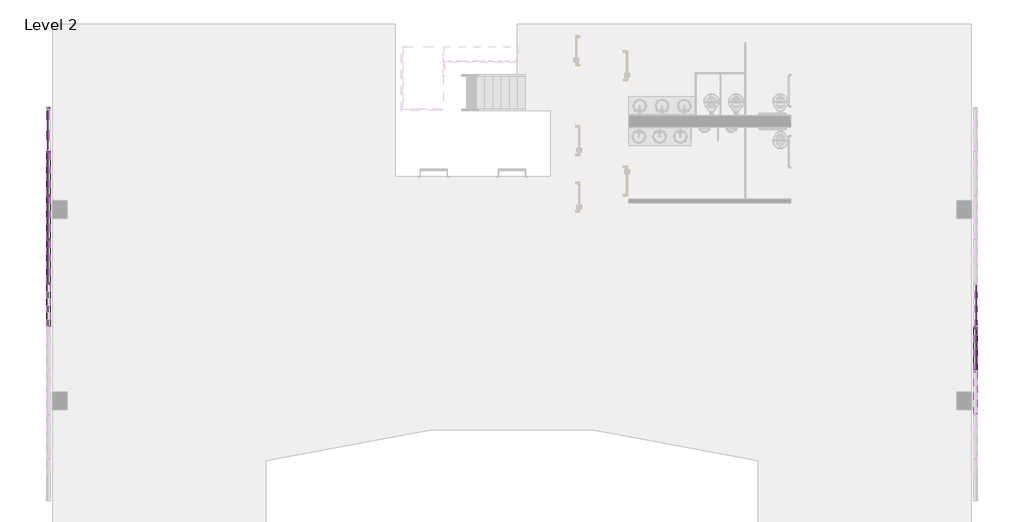
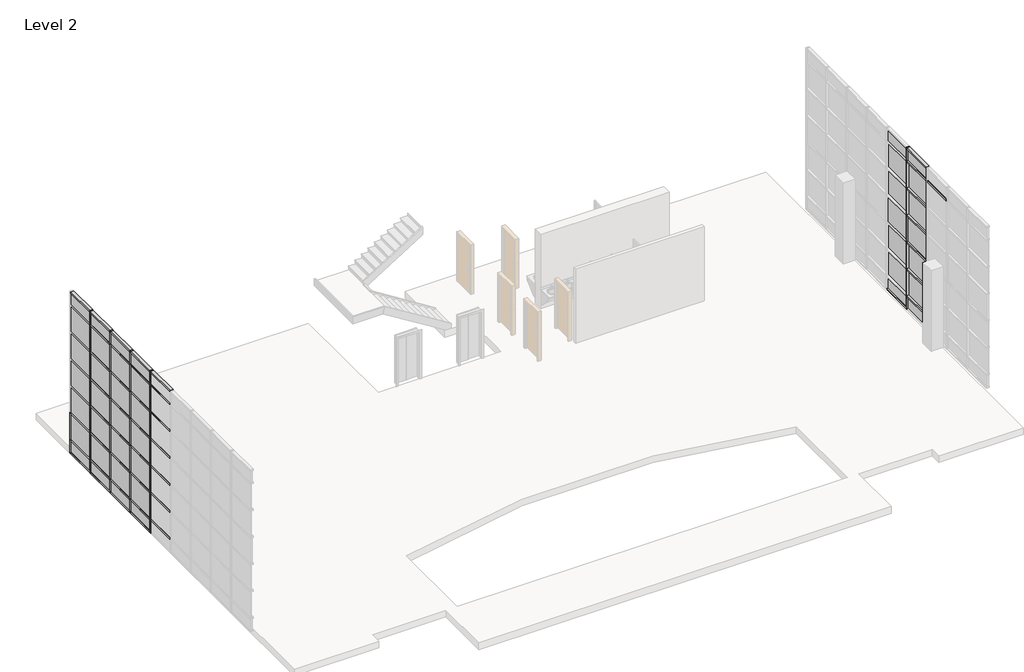
# One storey, part 4 of 6: 79 members, 42 plates.
"""IFC4 building model written with IfcOpenShell, lengths in millimetres."""

import ifcopenshell
import ifcopenshell.guid

model = None  # the IFC model being written
_history = None  # IfcOwnerHistory: only IFC2X3 demands one
_inside = {}  # id of a spatial element -> (the spatial element, [elements in it])
_under = {}  # id of a project, library or spatial element -> (it, [spatial elements below it])
_declared = {}  # id of a project -> (the project, [libraries it declares])
_typed = {}  # id of a type object -> (the type object, [elements of that type])
_made_of = {}  # id of a material, layer set ... -> (it, [elements and type objects made of it])


def new_model(schema):
    """Start an empty IFC model of exactly this schema.

    Asked for "IFC4X3", IfcOpenShell would pick the latest addendum, in which some entities
    have other attributes; the version numbers below select the first issue.
    IFC2X3 requires an IfcOwnerHistory on every rooted entity: one is made here for all.
    """
    global model, _history
    if schema == "IFC4X3":
        model = ifcopenshell.file(schema_version=(4, 3, 0, 0))
    else:
        model = ifcopenshell.file(schema=schema)
    _inside.clear()
    _under.clear()
    _declared.clear()
    _typed.clear()
    _made_of.clear()
    _history = None
    if model.schema == "IFC2X3":
        org = make("IfcOrganization", Name="unknown")
        user = make(
            "IfcPersonAndOrganization",
            ThePerson=make("IfcPerson", FamilyName="unknown"),
            TheOrganization=org,
        )
        app = make(
            "IfcApplication",
            ApplicationDeveloper=org,
            Version="unknown",
            ApplicationFullName="unknown",
            ApplicationIdentifier="unknown",
        )
        _history = make(
            "IfcOwnerHistory",
            OwningUser=user,
            OwningApplication=app,
            ChangeAction="ADDED",
            CreationDate=0,
        )
    return model


def make(cls, **values):
    """One entity of the class cls with the attributes given. An attribute that is None is left unset."""
    return model.create_entity(
        cls, **{name: value for name, value in values.items() if value is not None}
    )


def rooted(cls, **values):
    """An entity with a GlobalId (a new one), such as an element, a storey or a relation."""
    return make(cls, GlobalId=ifcopenshell.guid.new(), OwnerHistory=_history, **values)


def si_unit(unit_type, name, prefix=None):
    """IfcSIUnit, for example si_unit("LENGTHUNIT", "METRE", prefix="MILLI")."""
    return make("IfcSIUnit", UnitType=unit_type, Prefix=prefix, Name=name)


def assignment(units):
    """IfcUnitAssignment: the units of a project."""
    return None if units is None else make("IfcUnitAssignment", Units=units)


def point(xyz):
    """IfcCartesianPoint."""
    return None if xyz is None else make("IfcCartesianPoint", Coordinates=xyz)


def direction(xyz):
    """IfcDirection."""
    return None if xyz is None else make("IfcDirection", DirectionRatios=xyz)


def frame(location, z_axis=None, x_axis=None):
    """IfcAxis2Placement3D, a coordinate frame: its origin and axes. An axis left out is left unset."""
    return make(
        "IfcAxis2Placement3D",
        Location=point(location),
        Axis=direction(z_axis),
        RefDirection=direction(x_axis),
    )


def origin():
    """The frame at (0, 0, 0) with its axes left unset."""
    return frame((0.0, 0.0, 0.0))


def origin_with_axes():
    """The frame at (0, 0, 0) with the z axis (0, 0, 1) and the x axis (1, 0, 0) written out."""
    return frame((0.0, 0.0, 0.0), z_axis=(0.0, 0.0, 1.0), x_axis=(1.0, 0.0, 0.0))


def place(relative_to, where):
    """IfcLocalPlacement: puts the frame where relative to a parent placement (None: the world)."""
    return make(
        "IfcLocalPlacement", PlacementRelTo=relative_to, RelativePlacement=where
    )


def context(
    kind, dimensions, precision=None, world=None, true_north=None, identifier=None
):
    """IfcGeometricRepresentationContext, for example the 3D "Model" context."""
    return make(
        "IfcGeometricRepresentationContext",
        ContextIdentifier=identifier,
        ContextType=kind,
        CoordinateSpaceDimension=dimensions,
        Precision=precision,
        WorldCoordinateSystem=world,
        TrueNorth=true_north,
    )


def project(units=None, contexts=None):
    """IfcProject with its units and contexts."""
    return rooted(
        "IfcProject",
        Name="project",
        RepresentationContexts=contexts,
        UnitsInContext=assignment(units),
    )


def spatial(cls, under=None, at=None, **own):
    """A site, building, storey or space (cls), placed at a placement, below another one or the project."""
    s = rooted(cls, ObjectPlacement=at, **own)
    if under is not None:
        _under.setdefault(under.id(), (under, []))[1].append(s)
    return s


def polyline(points):
    """IfcPolyline through the points."""
    return make("IfcPolyline", Points=[point(p) for p in points])


def outline(outer, holes=None, kind="AREA"):
    """IfcArbitraryClosedProfileDef: a profile drawn as a closed curve; with holes, ...WithVoids."""
    if holes is None:
        return make("IfcArbitraryClosedProfileDef", ProfileType=kind, OuterCurve=outer)
    return make(
        "IfcArbitraryProfileDefWithVoids",
        ProfileType=kind,
        OuterCurve=outer,
        InnerCurves=holes,
    )


def extrude(swept, where, along, depth):
    """IfcExtrudedAreaSolid: the profile swept, set in the frame where, extruded along a direction by depth."""
    return make(
        "IfcExtrudedAreaSolid",
        SweptArea=swept,
        Position=where,
        ExtrudedDirection=direction(along),
        Depth=depth,
    )


def shape(context_of_items, identifier, shape_type, items):
    """IfcShapeRepresentation: the items that make up one representation, for example the "Body"."""
    return make(
        "IfcShapeRepresentation",
        ContextOfItems=context_of_items,
        RepresentationIdentifier=identifier,
        RepresentationType=shape_type,
        Items=items,
    )


def source(mapping_origin, context_of_items, identifier, shape_type, items):
    """IfcRepresentationMap: a shape defined once, which mapped items show again and again."""
    return make(
        "IfcRepresentationMap",
        MappingOrigin=mapping_origin,
        MappedRepresentation=shape(context_of_items, identifier, shape_type, items),
    )


def transform(
    local_origin,
    x_axis=None,
    y_axis=None,
    z_axis=None,
    scale=None,
    scale2=None,
    scale3=None,
    uniform=True,
):
    """IfcCartesianTransformationOperator3D, or its non-uniform kind. x_axis, y_axis, z_axis: its Axis1, 2, 3."""
    if uniform:
        return make(
            "IfcCartesianTransformationOperator3D",
            Axis1=direction(x_axis),
            Axis2=direction(y_axis),
            LocalOrigin=point(local_origin),
            Scale=scale,
            Axis3=direction(z_axis),
        )
    return make(
        "IfcCartesianTransformationOperator3DnonUniform",
        Axis1=direction(x_axis),
        Axis2=direction(y_axis),
        LocalOrigin=point(local_origin),
        Scale=scale,
        Axis3=direction(z_axis),
        Scale2=scale2,
        Scale3=scale3,
    )


def mapped(mapping_source, mapping_target):
    """IfcMappedItem: shows the shape of a source again, moved by a transform."""
    return make(
        "IfcMappedItem", MappingSource=mapping_source, MappingTarget=mapping_target
    )


def made_of(thing, what):
    """Note that an element or type object is made of a material, layer set ...; save() writes the relation."""
    if what is not None:
        _made_of.setdefault(what.id(), (what, []))[1].append(thing)
    return thing


def element(
    cls,
    number,
    at=None,
    inside=None,
    cuts=None,
    type_object=None,
    material=None,
    context=None,
    identifier="Body",
    shape_type=None,
    held_by="IfcProductDefinitionShape",
    body=None,
    shapes=None,
    **own,
):
    """One element of the class cls, such as IfcWall. Its Tag is "e" and its number.

    at: its placement. inside: the storey or other place that contains it. cuts: it is an
    opening in that element (IfcRelVoidsElement). A single representation is given by context,
    identifier, shape_type and body (its items); several are given by shapes. held_by: the class
    of the entity that holds the representations. save() writes the other relations.
    """
    e = rooted(cls, Tag="e%d" % number, ObjectPlacement=at, **own)
    if body is not None:
        shapes = [shape(context, identifier, shape_type, body)]
    if shapes is not None:
        e.Representation = make(held_by, Representations=shapes)
    if inside is not None:
        _inside.setdefault(inside.id(), (inside, []))[1].append(e)
    if cuts is not None:
        rooted(
            "IfcRelVoidsElement", RelatingBuildingElement=cuts, RelatedOpeningElement=e
        )
    if type_object is not None:
        _typed.setdefault(type_object.id(), (type_object, []))[1].append(e)
    return made_of(e, material)


def aggregate(whole, parts):
    """IfcRelAggregates: a whole, such as a stair, and the parts it consists of."""
    return rooted("IfcRelAggregates", RelatingObject=whole, RelatedObjects=parts)


def save(model, path):
    """Write the relations noted so far, then the file.

    IfcRelAggregates (storeys below a building ...), IfcRelContainedInSpatialStructure (elements
    in a storey), IfcRelDefinesByType, IfcRelAssociatesMaterial and IfcRelDeclares: one each for
    every whole, place, type object, material and project.
    """
    for whole, parts in _under.values():
        aggregate(whole, parts)
    for where, things in _inside.values():
        rooted(
            "IfcRelContainedInSpatialStructure",
            RelatedElements=things,
            RelatingStructure=where,
        )
    for kind, things in _typed.values():
        rooted("IfcRelDefinesByType", RelatedObjects=things, RelatingType=kind)
    for what, things in _made_of.values():
        rooted("IfcRelAssociatesMaterial", RelatedObjects=things, RelatingMaterial=what)
    for by, libraries in _declared.values():
        rooted("IfcRelDeclares", RelatingContext=by, RelatedDefinitions=libraries)
    model.write(path)


def member_7b0bb32c(model_context):
    return source(origin(), model_context, "Body", "SweptSolid", [
        extrude(outline(polyline([(0.0, 63.5), (0.0, -63.5), (-63.5, -63.5), (-63.5, 63.5), (0.0, 63.5)])), frame((0.0, 0.0, -1394.8833336), z_axis=(0.0, 0.0, 1.0), x_axis=(1.0, 0.0, 0.0)), (0.0, 0.0, 1.0), 1394.8833336),
    ])


def member_2e151cea(model_context):
    return source(origin(), model_context, "Body", "SweptSolid", [
        extrude(outline(polyline([(0.0, 63.5), (0.0, -63.5), (-63.5, -63.5), (-63.5, 63.5), (0.0, 63.5)])), frame((0.0, 0.0, -1426.6333333), z_axis=(0.0, 0.0, 1.0), x_axis=(1.0, 0.0, 0.0)), (0.0, 0.0, 1.0), 1426.6333333),
    ])


def member_3c30aa5e(model_context):
    return source(origin(), model_context, "Body", "SweptSolid", [
        extrude(outline(polyline([(31.75, 63.5), (31.75, -63.5), (-31.75, -63.5), (-31.75, 63.5), (31.75, 63.5)])), frame((0.0, 0.0, -1426.6333333), z_axis=(0.0, 0.0, 1.0), x_axis=(1.0, 0.0, 0.0)), (0.0, 0.0, 1.0), 1426.6333333),
    ])


def member_2b49869a(model_context):
    return source(origin(), model_context, "Body", "SweptSolid", [
        extrude(outline(polyline([(31.75, 63.5), (31.75, -63.5), (-31.75, -63.5), (-31.75, 63.5), (31.75, 63.5)])), frame((0.0, 0.0, -1219.2), z_axis=(0.0, 0.0, 1.0), x_axis=(1.0, 0.0, 0.0)), (0.0, 0.0, 1.0), 1219.2),
    ])


def member_75074519(model_context):
    return source(origin(), model_context, "Body", "SweptSolid", [
        extrude(outline(polyline([(0.0, 63.5), (0.0, -63.5), (-63.5, -63.5), (-63.5, 63.5), (0.0, 63.5)])), frame((0.0, 0.0, -1219.2), z_axis=(0.0, 0.0, 1.0), x_axis=(1.0, 0.0, 0.0)), (0.0, 0.0, 1.0), 1219.2),
    ])


def member_6e77e263(model_context):
    return source(origin(), model_context, "Body", "SweptSolid", [
        extrude(outline(polyline([(31.75, 63.5), (31.75, -63.5), (-31.75, -63.5), (-31.75, 63.5), (31.75, 63.5)])), frame((0.0, 0.0, -609.6), z_axis=(0.0, 0.0, 1.0), x_axis=(1.0, 0.0, 0.0)), (0.0, 0.0, 1.0), 609.6),
    ])


def member_47bfaf8a(model_context):
    return source(origin(), model_context, "Body", "SweptSolid", [
        extrude(outline(polyline([(0.0, 63.5), (0.0, -63.5), (-63.5, -63.5), (-63.5, 63.5), (0.0, 63.5)])), frame((0.0, 0.0, -609.6), z_axis=(0.0, 0.0, 1.0), x_axis=(1.0, 0.0, 0.0)), (0.0, 0.0, 1.0), 609.6),
    ])


def system_panel_glazed_88b4eb2b(model_context):
    return source(origin(), model_context, "Body", "SweptSolid", [
        extrude(outline(polyline([(697.4416668, 19.05), (-697.4416668, 19.05), (-697.4416668, 44.45), (697.4416668, 44.45), (697.4416668, 19.05)])), origin_with_axes(), (0.0, 0.0, 1.0), 1155.7),
    ])


def system_panel_glazed_8e8b8cb0(model_context):
    return source(origin(), model_context, "Body", "SweptSolid", [
        extrude(outline(polyline([(713.3166666, 19.05), (-713.3166666, 19.05), (-713.3166666, 44.45), (713.3166666, 44.45), (713.3166666, 19.05)])), origin_with_axes(), (0.0, 0.0, 1.0), 1155.7),
    ])


def system_panel_glazed_0adb819a(model_context):
    return source(origin(), model_context, "Body", "SweptSolid", [
        extrude(outline(polyline([(713.3166666, -44.45), (-713.3166666, -44.45), (-713.3166666, -19.05), (713.3166666, -19.05), (713.3166666, -44.45)])), origin_with_axes(), (0.0, 0.0, 1.0), 1155.7),
    ])


def system_panel_solid_8f383511(model_context):
    return source(origin(), model_context, "Body", "SweptSolid", [
        extrude(outline(polyline([(697.4416668, -19.05), (-697.4416668, -19.05), (-697.4416668, 44.45), (697.4416668, 44.45), (697.4416668, -19.05)])), origin_with_axes(), (0.0, 0.0, 1.0), 1155.7),
    ])


def system_panel_solid_81e17396(model_context):
    return source(origin(), model_context, "Body", "SweptSolid", [
        extrude(outline(polyline([(713.3166666, -19.05), (-713.3166666, -19.05), (-713.3166666, 44.45), (713.3166666, 44.45), (713.3166666, -19.05)])), origin_with_axes(), (0.0, 0.0, 1.0), 1155.7),
    ])


def system_panel_solid_21827ae2(model_context):
    return source(origin(), model_context, "Body", "SweptSolid", [
        extrude(outline(polyline([(697.4416668, -19.05), (-697.4416668, -19.05), (-697.4416668, 44.45), (697.4416668, 44.45), (697.4416668, -19.05)])), origin_with_axes(), (0.0, 0.0, 1.0), 514.35),
    ])


def system_panel_solid_4932440a(model_context):
    return source(origin(), model_context, "Body", "SweptSolid", [
        extrude(outline(polyline([(713.3166666, -19.05), (-713.3166666, -19.05), (-713.3166666, 44.45), (713.3166666, 44.45), (713.3166666, -19.05)])), origin_with_axes(), (0.0, 0.0, 1.0), 514.35),
    ])


def system_panel_solid_81598777(model_context):
    return source(origin(), model_context, "Body", "SweptSolid", [
        extrude(outline(polyline([(713.3166666, -44.45), (-713.3166666, -44.45), (-713.3166666, 19.05), (713.3166666, 19.05), (713.3166666, -44.45)])), origin_with_axes(), (0.0, 0.0, 1.0), 514.35),
    ])


def system_panel_solid_db88bede(model_context):
    return source(origin(), model_context, "Body", "SweptSolid", [
        extrude(outline(polyline([(713.3166666, -44.45), (-713.3166666, -44.45), (-713.3166666, 19.05), (713.3166666, 19.05), (713.3166666, -44.45)])), origin_with_axes(), (0.0, 0.0, 1.0), 1155.7),
    ])


model = new_model("IFC4")

# Units and contexts
model_context = context("Model", 3, world=origin())
ifc_project = project(units=[si_unit("LENGTHUNIT", "METRE", prefix="MILLI")], contexts=[model_context])

# Site, building, storey
site = spatial("IfcSite", under=ifc_project)
building = spatial("IfcBuilding", under=site)
storey = spatial("IfcBuildingStorey", under=building, Name="Level 2", Elevation=3657.6)

# Members
placement = place(None, origin())
member_shape = member_7b0bb32c(model_context)
element("IfcMember", 1, ObjectType="Rectangular Mullion : 2.5\" x 5\" rectangular", at=placement, inside=storey, context=model_context, shape_type="MappedRepresentation", body=[
    mapped(member_shape, transform((-16888.4122732, 6484.8015304, 10972.8), x_axis=(0.0, 0.0, 1.0), y_axis=(1.0, 0.0, 0.0), z_axis=(0.0, 1.0, 0.0))),
])
member_2_shape = member_2e151cea(model_context)
element("IfcMember", 2, ObjectType="Rectangular Mullion : 2.5\" x 5\" rectangular", at=placement, inside=storey, context=model_context, shape_type="MappedRepresentation", body=[
    mapped(member_2_shape, transform((-16888.4122732, 556.018197, 10972.8), x_axis=(0.0, 0.0, 1.0), y_axis=(1.0, 0.0, 0.0), z_axis=(0.0, 1.0, 0.0))),
])
element("IfcMember", 3, ObjectType="Rectangular Mullion : 2.5\" x 5\" rectangular", at=placement, inside=storey, context=model_context, shape_type="MappedRepresentation", body=[
    mapped(member_2_shape, transform((-16888.4122732, 2046.1515303, 10972.8), x_axis=(0.0, 0.0, 1.0), y_axis=(1.0, 0.0, 0.0), z_axis=(0.0, 1.0, 0.0))),
])
element("IfcMember", 4, ObjectType="Rectangular Mullion : 2.5\" x 5\" rectangular", at=placement, inside=storey, context=model_context, shape_type="MappedRepresentation", body=[
    mapped(member_2_shape, transform((-16888.4122732, 3536.2848635, 10972.8), x_axis=(0.0, 0.0, 1.0), y_axis=(1.0, 0.0, 0.0), z_axis=(0.0, 1.0, 0.0))),
])
element("IfcMember", 5, ObjectType="Rectangular Mullion : 2.5\" x 5\" rectangular", at=placement, inside=storey, context=model_context, shape_type="MappedRepresentation", body=[
    mapped(member_2_shape, transform((-16888.4122732, 5026.4181968, 10972.8), x_axis=(0.0, 0.0, 1.0), y_axis=(1.0, 0.0, 0.0), z_axis=(0.0, 1.0, 0.0))),
])
element("IfcMember", 6, ObjectType="Rectangular Mullion : 2.5\" x 5\" rectangular", at=placement, inside=storey, context=model_context, shape_type="MappedRepresentation", body=[
    mapped(member_shape, transform((-16888.4122732, 5089.9181968, 3657.6), x_axis=(0.0, 0.0, -1.0), y_axis=(1.0, 0.0, 0.0), z_axis=(0.0, -1.0, 0.0))),
])
element("IfcMember", 7, ObjectType="Rectangular Mullion : 2.5\" x 5\" rectangular", at=placement, inside=storey, context=model_context, shape_type="MappedRepresentation", body=[
    mapped(member_2_shape, transform((-16888.4122732, 619.518197, 3657.6), x_axis=(0.0, 0.0, -1.0), y_axis=(1.0, 0.0, 0.0), z_axis=(0.0, -1.0, 0.0))),
])
element("IfcMember", 8, ObjectType="Rectangular Mullion : 2.5\" x 5\" rectangular", at=placement, inside=storey, context=model_context, shape_type="MappedRepresentation", body=[
    mapped(member_2_shape, transform((-16888.4122732, 2109.6515303, 3657.6), x_axis=(0.0, 0.0, -1.0), y_axis=(1.0, 0.0, 0.0), z_axis=(0.0, -1.0, 0.0))),
])
element("IfcMember", 9, ObjectType="Rectangular Mullion : 2.5\" x 5\" rectangular", at=placement, inside=storey, context=model_context, shape_type="MappedRepresentation", body=[
    mapped(member_2_shape, transform((-16888.4122732, 3599.7848635, 3657.6), x_axis=(0.0, 0.0, -1.0), y_axis=(1.0, 0.0, 0.0), z_axis=(0.0, -1.0, 0.0))),
])
member_3_shape = member_3c30aa5e(model_context)
element("IfcMember", 10, ObjectType="Rectangular Mullion : 2.5\" x 5\" rectangular", at=placement, inside=storey, context=model_context, shape_type="MappedRepresentation", body=[
    mapped(member_3_shape, transform((-16888.4122732, 556.018197, 4267.2), x_axis=(0.0, 0.0, 1.0), y_axis=(1.0, 0.0, 0.0), z_axis=(0.0, 1.0, 0.0))),
])
element("IfcMember", 11, ObjectType="Rectangular Mullion : 2.5\" x 5\" rectangular", at=placement, inside=storey, context=model_context, shape_type="MappedRepresentation", body=[
    mapped(member_3_shape, transform((-16888.4122732, 2046.1515303, 4267.2), x_axis=(0.0, 0.0, 1.0), y_axis=(1.0, 0.0, 0.0), z_axis=(0.0, 1.0, 0.0))),
])
element("IfcMember", 12, ObjectType="Rectangular Mullion : 2.5\" x 5\" rectangular", at=placement, inside=storey, context=model_context, shape_type="MappedRepresentation", body=[
    mapped(member_3_shape, transform((-16888.4122732, 3536.2848635, 4267.2), x_axis=(0.0, 0.0, 1.0), y_axis=(1.0, 0.0, 0.0), z_axis=(0.0, 1.0, 0.0))),
])
element("IfcMember", 13, ObjectType="Rectangular Mullion : 2.5\" x 5\" rectangular", at=placement, inside=storey, context=model_context, shape_type="MappedRepresentation", body=[
    mapped(member_3_shape, transform((-16888.4122732, 5026.4181968, 4267.2), x_axis=(0.0, 0.0, 1.0), y_axis=(1.0, 0.0, 0.0), z_axis=(0.0, 1.0, 0.0))),
])
element("IfcMember", 14, ObjectType="Rectangular Mullion : 2.5\" x 5\" rectangular", at=placement, inside=storey, context=model_context, shape_type="MappedRepresentation", body=[
    mapped(member_3_shape, transform((-16888.4122732, 556.018197, 5486.4), x_axis=(0.0, 0.0, 1.0), y_axis=(1.0, 0.0, 0.0), z_axis=(0.0, 1.0, 0.0))),
])
element("IfcMember", 15, ObjectType="Rectangular Mullion : 2.5\" x 5\" rectangular", at=placement, inside=storey, context=model_context, shape_type="MappedRepresentation", body=[
    mapped(member_3_shape, transform((-16888.4122732, 2046.1515303, 5486.4), x_axis=(0.0, 0.0, 1.0), y_axis=(1.0, 0.0, 0.0), z_axis=(0.0, 1.0, 0.0))),
])
element("IfcMember", 16, ObjectType="Rectangular Mullion : 2.5\" x 5\" rectangular", at=placement, inside=storey, context=model_context, shape_type="MappedRepresentation", body=[
    mapped(member_3_shape, transform((-16888.4122732, 3536.2848635, 5486.4), x_axis=(0.0, 0.0, 1.0), y_axis=(1.0, 0.0, 0.0), z_axis=(0.0, 1.0, 0.0))),
])
element("IfcMember", 17, ObjectType="Rectangular Mullion : 2.5\" x 5\" rectangular", at=placement, inside=storey, context=model_context, shape_type="MappedRepresentation", body=[
    mapped(member_3_shape, transform((-16888.4122732, 5026.4181968, 5486.4), x_axis=(0.0, 0.0, 1.0), y_axis=(1.0, 0.0, 0.0), z_axis=(0.0, 1.0, 0.0))),
])
element("IfcMember", 18, ObjectType="Rectangular Mullion : 2.5\" x 5\" rectangular", at=placement, inside=storey, context=model_context, shape_type="MappedRepresentation", body=[
    mapped(member_3_shape, transform((-16888.4122732, 556.018197, 6705.6), x_axis=(0.0, 0.0, 1.0), y_axis=(1.0, 0.0, 0.0), z_axis=(0.0, 1.0, 0.0))),
])
element("IfcMember", 19, ObjectType="Rectangular Mullion : 2.5\" x 5\" rectangular", at=placement, inside=storey, context=model_context, shape_type="MappedRepresentation", body=[
    mapped(member_3_shape, transform((-16888.4122732, 2046.1515303, 6705.6), x_axis=(0.0, 0.0, 1.0), y_axis=(1.0, 0.0, 0.0), z_axis=(0.0, 1.0, 0.0))),
])
element("IfcMember", 20, ObjectType="Rectangular Mullion : 2.5\" x 5\" rectangular", at=placement, inside=storey, context=model_context, shape_type="MappedRepresentation", body=[
    mapped(member_3_shape, transform((-16888.4122732, 3536.2848635, 6705.6), x_axis=(0.0, 0.0, 1.0), y_axis=(1.0, 0.0, 0.0), z_axis=(0.0, 1.0, 0.0))),
])
element("IfcMember", 21, ObjectType="Rectangular Mullion : 2.5\" x 5\" rectangular", at=placement, inside=storey, context=model_context, shape_type="MappedRepresentation", body=[
    mapped(member_3_shape, transform((-16888.4122732, 5026.4181968, 6705.6), x_axis=(0.0, 0.0, 1.0), y_axis=(1.0, 0.0, 0.0), z_axis=(0.0, 1.0, 0.0))),
])
element("IfcMember", 22, ObjectType="Rectangular Mullion : 2.5\" x 5\" rectangular", at=placement, inside=storey, context=model_context, shape_type="MappedRepresentation", body=[
    mapped(member_3_shape, transform((-16888.4122732, 556.018197, 7924.8), x_axis=(0.0, 0.0, 1.0), y_axis=(1.0, 0.0, 0.0), z_axis=(0.0, 1.0, 0.0))),
])
element("IfcMember", 23, ObjectType="Rectangular Mullion : 2.5\" x 5\" rectangular", at=placement, inside=storey, context=model_context, shape_type="MappedRepresentation", body=[
    mapped(member_3_shape, transform((-16888.4122732, 2046.1515303, 7924.8), x_axis=(0.0, 0.0, 1.0), y_axis=(1.0, 0.0, 0.0), z_axis=(0.0, 1.0, 0.0))),
])
element("IfcMember", 24, ObjectType="Rectangular Mullion : 2.5\" x 5\" rectangular", at=placement, inside=storey, context=model_context, shape_type="MappedRepresentation", body=[
    mapped(member_3_shape, transform((-16888.4122732, 3536.2848635, 7924.8), x_axis=(0.0, 0.0, 1.0), y_axis=(1.0, 0.0, 0.0), z_axis=(0.0, 1.0, 0.0))),
])
element("IfcMember", 25, ObjectType="Rectangular Mullion : 2.5\" x 5\" rectangular", at=placement, inside=storey, context=model_context, shape_type="MappedRepresentation", body=[
    mapped(member_3_shape, transform((-16888.4122732, 5026.4181968, 7924.8), x_axis=(0.0, 0.0, 1.0), y_axis=(1.0, 0.0, 0.0), z_axis=(0.0, 1.0, 0.0))),
])
element("IfcMember", 26, ObjectType="Rectangular Mullion : 2.5\" x 5\" rectangular", at=placement, inside=storey, context=model_context, shape_type="MappedRepresentation", body=[
    mapped(member_3_shape, transform((-16888.4122732, 556.018197, 9144.0), x_axis=(0.0, 0.0, 1.0), y_axis=(1.0, 0.0, 0.0), z_axis=(0.0, 1.0, 0.0))),
])
element("IfcMember", 27, ObjectType="Rectangular Mullion : 2.5\" x 5\" rectangular", at=placement, inside=storey, context=model_context, shape_type="MappedRepresentation", body=[
    mapped(member_3_shape, transform((-16888.4122732, 2046.1515303, 9144.0), x_axis=(0.0, 0.0, 1.0), y_axis=(1.0, 0.0, 0.0), z_axis=(0.0, 1.0, 0.0))),
])
element("IfcMember", 28, ObjectType="Rectangular Mullion : 2.5\" x 5\" rectangular", at=placement, inside=storey, context=model_context, shape_type="MappedRepresentation", body=[
    mapped(member_3_shape, transform((-16888.4122732, 3536.2848635, 9144.0), x_axis=(0.0, 0.0, 1.0), y_axis=(1.0, 0.0, 0.0), z_axis=(0.0, 1.0, 0.0))),
])
element("IfcMember", 29, ObjectType="Rectangular Mullion : 2.5\" x 5\" rectangular", at=placement, inside=storey, context=model_context, shape_type="MappedRepresentation", body=[
    mapped(member_3_shape, transform((-16888.4122732, 5026.4181968, 9144.0), x_axis=(0.0, 0.0, 1.0), y_axis=(1.0, 0.0, 0.0), z_axis=(0.0, 1.0, 0.0))),
])
element("IfcMember", 30, ObjectType="Rectangular Mullion : 2.5\" x 5\" rectangular", at=placement, inside=storey, context=model_context, shape_type="MappedRepresentation", body=[
    mapped(member_3_shape, transform((-16888.4122732, 556.018197, 10363.2), x_axis=(0.0, 0.0, 1.0), y_axis=(1.0, 0.0, 0.0), z_axis=(0.0, 1.0, 0.0))),
])
element("IfcMember", 31, ObjectType="Rectangular Mullion : 2.5\" x 5\" rectangular", at=placement, inside=storey, context=model_context, shape_type="MappedRepresentation", body=[
    mapped(member_3_shape, transform((-16888.4122732, 2046.1515303, 10363.2), x_axis=(0.0, 0.0, 1.0), y_axis=(1.0, 0.0, 0.0), z_axis=(0.0, 1.0, 0.0))),
])
element("IfcMember", 32, ObjectType="Rectangular Mullion : 2.5\" x 5\" rectangular", at=placement, inside=storey, context=model_context, shape_type="MappedRepresentation", body=[
    mapped(member_3_shape, transform((-16888.4122732, 3536.2848635, 10363.2), x_axis=(0.0, 0.0, 1.0), y_axis=(1.0, 0.0, 0.0), z_axis=(0.0, 1.0, 0.0))),
])
element("IfcMember", 33, ObjectType="Rectangular Mullion : 2.5\" x 5\" rectangular", at=placement, inside=storey, context=model_context, shape_type="MappedRepresentation", body=[
    mapped(member_3_shape, transform((-16888.4122732, 5026.4181968, 10363.2), x_axis=(0.0, 0.0, 1.0), y_axis=(1.0, 0.0, 0.0), z_axis=(0.0, 1.0, 0.0))),
])
member_4_shape = member_2b49869a(model_context)
element("IfcMember", 34, ObjectType="Rectangular Mullion : 2.5\" x 5\" rectangular", at=placement, inside=storey, context=model_context, shape_type="MappedRepresentation", body=[
    mapped(member_4_shape, transform((-16888.4122732, 587.768197, 4267.2), x_axis=(0.0, 1.0, 0.0), y_axis=(1.0, 0.0, 0.0), z_axis=(0.0, 0.0, -1.0))),
])
element("IfcMember", 35, ObjectType="Rectangular Mullion : 2.5\" x 5\" rectangular", at=placement, inside=storey, context=model_context, shape_type="MappedRepresentation", body=[
    mapped(member_4_shape, transform((-16888.4122732, 2077.9015303, 4267.2), x_axis=(0.0, 1.0, 0.0), y_axis=(1.0, 0.0, 0.0), z_axis=(0.0, 0.0, -1.0))),
])
element("IfcMember", 36, ObjectType="Rectangular Mullion : 2.5\" x 5\" rectangular", at=placement, inside=storey, context=model_context, shape_type="MappedRepresentation", body=[
    mapped(member_4_shape, transform((-16888.4122732, 3568.0348635, 4267.2), x_axis=(0.0, 1.0, 0.0), y_axis=(1.0, 0.0, 0.0), z_axis=(0.0, 0.0, -1.0))),
])
element("IfcMember", 37, ObjectType="Rectangular Mullion : 2.5\" x 5\" rectangular", at=placement, inside=storey, context=model_context, shape_type="MappedRepresentation", body=[
    mapped(member_4_shape, transform((-16888.4122732, 5058.1681968, 4267.2), x_axis=(0.0, 1.0, 0.0), y_axis=(1.0, 0.0, 0.0), z_axis=(0.0, 0.0, -1.0))),
])
element("IfcMember", 38, ObjectType="Rectangular Mullion : 2.5\" x 5\" rectangular", at=placement, inside=storey, context=model_context, shape_type="MappedRepresentation", body=[
    mapped(member_4_shape, transform((-16888.4122732, 587.768197, 5486.4), x_axis=(0.0, 1.0, 0.0), y_axis=(1.0, 0.0, 0.0), z_axis=(0.0, 0.0, -1.0))),
])
element("IfcMember", 39, ObjectType="Rectangular Mullion : 2.5\" x 5\" rectangular", at=placement, inside=storey, context=model_context, shape_type="MappedRepresentation", body=[
    mapped(member_4_shape, transform((-16888.4122732, 2077.9015303, 5486.4), x_axis=(0.0, 1.0, 0.0), y_axis=(1.0, 0.0, 0.0), z_axis=(0.0, 0.0, -1.0))),
])
element("IfcMember", 40, ObjectType="Rectangular Mullion : 2.5\" x 5\" rectangular", at=placement, inside=storey, context=model_context, shape_type="MappedRepresentation", body=[
    mapped(member_4_shape, transform((-16888.4122732, 3568.0348635, 5486.4), x_axis=(0.0, 1.0, 0.0), y_axis=(1.0, 0.0, 0.0), z_axis=(0.0, 0.0, -1.0))),
])
element("IfcMember", 41, ObjectType="Rectangular Mullion : 2.5\" x 5\" rectangular", at=placement, inside=storey, context=model_context, shape_type="MappedRepresentation", body=[
    mapped(member_4_shape, transform((-16888.4122732, 5058.1681968, 5486.4), x_axis=(0.0, 1.0, 0.0), y_axis=(1.0, 0.0, 0.0), z_axis=(0.0, 0.0, -1.0))),
])
element("IfcMember", 42, ObjectType="Rectangular Mullion : 2.5\" x 5\" rectangular", at=placement, inside=storey, context=model_context, shape_type="MappedRepresentation", body=[
    mapped(member_4_shape, transform((-16888.4122732, 587.768197, 6705.6), x_axis=(0.0, 1.0, 0.0), y_axis=(1.0, 0.0, 0.0), z_axis=(0.0, 0.0, -1.0))),
])
element("IfcMember", 43, ObjectType="Rectangular Mullion : 2.5\" x 5\" rectangular", at=placement, inside=storey, context=model_context, shape_type="MappedRepresentation", body=[
    mapped(member_4_shape, transform((-16888.4122732, 587.768197, 7924.8), x_axis=(0.0, 1.0, 0.0), y_axis=(1.0, 0.0, 0.0), z_axis=(0.0, 0.0, -1.0))),
])
element("IfcMember", 44, ObjectType="Rectangular Mullion : 2.5\" x 5\" rectangular", at=placement, inside=storey, context=model_context, shape_type="MappedRepresentation", body=[
    mapped(member_4_shape, transform((-16888.4122732, 587.768197, 9144.0), x_axis=(0.0, 1.0, 0.0), y_axis=(1.0, 0.0, 0.0), z_axis=(0.0, 0.0, -1.0))),
])
element("IfcMember", 45, ObjectType="Rectangular Mullion : 2.5\" x 5\" rectangular", at=placement, inside=storey, context=model_context, shape_type="MappedRepresentation", body=[
    mapped(member_4_shape, transform((-16888.4122732, 2077.9015303, 6705.6), x_axis=(0.0, 1.0, 0.0), y_axis=(1.0, 0.0, 0.0), z_axis=(0.0, 0.0, -1.0))),
])
element("IfcMember", 46, ObjectType="Rectangular Mullion : 2.5\" x 5\" rectangular", at=placement, inside=storey, context=model_context, shape_type="MappedRepresentation", body=[
    mapped(member_4_shape, transform((-16888.4122732, 2077.9015303, 7924.8), x_axis=(0.0, 1.0, 0.0), y_axis=(1.0, 0.0, 0.0), z_axis=(0.0, 0.0, -1.0))),
])
element("IfcMember", 47, ObjectType="Rectangular Mullion : 2.5\" x 5\" rectangular", at=placement, inside=storey, context=model_context, shape_type="MappedRepresentation", body=[
    mapped(member_4_shape, transform((-16888.4122732, 2077.9015303, 9144.0), x_axis=(0.0, 1.0, 0.0), y_axis=(1.0, 0.0, 0.0), z_axis=(0.0, 0.0, -1.0))),
])
element("IfcMember", 48, ObjectType="Rectangular Mullion : 2.5\" x 5\" rectangular", at=placement, inside=storey, context=model_context, shape_type="MappedRepresentation", body=[
    mapped(member_4_shape, transform((-16888.4122732, 3568.0348635, 6705.6), x_axis=(0.0, 1.0, 0.0), y_axis=(1.0, 0.0, 0.0), z_axis=(0.0, 0.0, -1.0))),
])
element("IfcMember", 49, ObjectType="Rectangular Mullion : 2.5\" x 5\" rectangular", at=placement, inside=storey, context=model_context, shape_type="MappedRepresentation", body=[
    mapped(member_4_shape, transform((-16888.4122732, 3568.0348635, 7924.8), x_axis=(0.0, 1.0, 0.0), y_axis=(1.0, 0.0, 0.0), z_axis=(0.0, 0.0, -1.0))),
])
element("IfcMember", 50, ObjectType="Rectangular Mullion : 2.5\" x 5\" rectangular", at=placement, inside=storey, context=model_context, shape_type="MappedRepresentation", body=[
    mapped(member_4_shape, transform((-16888.4122732, 3568.0348635, 9144.0), x_axis=(0.0, 1.0, 0.0), y_axis=(1.0, 0.0, 0.0), z_axis=(0.0, 0.0, -1.0))),
])
element("IfcMember", 51, ObjectType="Rectangular Mullion : 2.5\" x 5\" rectangular", at=placement, inside=storey, context=model_context, shape_type="MappedRepresentation", body=[
    mapped(member_4_shape, transform((-16888.4122732, 5058.1681968, 6705.6), x_axis=(0.0, 1.0, 0.0), y_axis=(1.0, 0.0, 0.0), z_axis=(0.0, 0.0, -1.0))),
])
element("IfcMember", 52, ObjectType="Rectangular Mullion : 2.5\" x 5\" rectangular", at=placement, inside=storey, context=model_context, shape_type="MappedRepresentation", body=[
    mapped(member_4_shape, transform((-16888.4122732, 5058.1681968, 7924.8), x_axis=(0.0, 1.0, 0.0), y_axis=(1.0, 0.0, 0.0), z_axis=(0.0, 0.0, -1.0))),
])
element("IfcMember", 53, ObjectType="Rectangular Mullion : 2.5\" x 5\" rectangular", at=placement, inside=storey, context=model_context, shape_type="MappedRepresentation", body=[
    mapped(member_4_shape, transform((-16888.4122732, 5058.1681968, 9144.0), x_axis=(0.0, 1.0, 0.0), y_axis=(1.0, 0.0, 0.0), z_axis=(0.0, 0.0, -1.0))),
])
member_5_shape = member_75074519(model_context)
element("IfcMember", 54, ObjectType="Rectangular Mullion : 2.5\" x 5\" rectangular", at=placement, inside=storey, context=model_context, shape_type="MappedRepresentation", body=[
    mapped(member_5_shape, transform((-16888.4122732, 6548.3015304, 4267.2), x_axis=(0.0, 1.0, 0.0), y_axis=(1.0, 0.0, 0.0), z_axis=(0.0, 0.0, -1.0))),
])
member_6_shape = member_6e77e263(model_context)
element("IfcMember", 55, ObjectType="Rectangular Mullion : 2.5\" x 5\" rectangular", at=placement, inside=storey, context=model_context, shape_type="MappedRepresentation", body=[
    mapped(member_6_shape, transform((-16888.4122732, 587.768197, 3657.6), x_axis=(0.0, 1.0, 0.0), y_axis=(1.0, 0.0, 0.0), z_axis=(0.0, 0.0, -1.0))),
])
element("IfcMember", 56, ObjectType="Rectangular Mullion : 2.5\" x 5\" rectangular", at=placement, inside=storey, context=model_context, shape_type="MappedRepresentation", body=[
    mapped(member_6_shape, transform((-16888.4122732, 2077.9015303, 3657.6), x_axis=(0.0, 1.0, 0.0), y_axis=(1.0, 0.0, 0.0), z_axis=(0.0, 0.0, -1.0))),
])
element("IfcMember", 57, ObjectType="Rectangular Mullion : 2.5\" x 5\" rectangular", at=placement, inside=storey, context=model_context, shape_type="MappedRepresentation", body=[
    mapped(member_6_shape, transform((-16888.4122732, 3568.0348635, 3657.6), x_axis=(0.0, 1.0, 0.0), y_axis=(1.0, 0.0, 0.0), z_axis=(0.0, 0.0, -1.0))),
])
element("IfcMember", 58, ObjectType="Rectangular Mullion : 2.5\" x 5\" rectangular", at=placement, inside=storey, context=model_context, shape_type="MappedRepresentation", body=[
    mapped(member_6_shape, transform((-16888.4122732, 5058.1681968, 3657.6), x_axis=(0.0, 1.0, 0.0), y_axis=(1.0, 0.0, 0.0), z_axis=(0.0, 0.0, -1.0))),
])
member_7_shape = member_47bfaf8a(model_context)
element("IfcMember", 59, ObjectType="Rectangular Mullion : 2.5\" x 5\" rectangular", at=placement, inside=storey, context=model_context, shape_type="MappedRepresentation", body=[
    mapped(member_7_shape, transform((-16888.4122732, 6548.3015304, 3657.6), x_axis=(0.0, 1.0, 0.0), y_axis=(1.0, 0.0, 0.0), z_axis=(0.0, 0.0, -1.0))),
])
element("IfcMember", 60, ObjectType="Rectangular Mullion : 2.5\" x 5\" rectangular", at=placement, inside=storey, context=model_context, shape_type="MappedRepresentation", body=[
    mapped(member_6_shape, transform((-16888.4122732, 587.768197, 10363.2), x_axis=(0.0, 1.0, 0.0), y_axis=(1.0, 0.0, 0.0), z_axis=(0.0, 0.0, -1.0))),
])
element("IfcMember", 61, ObjectType="Rectangular Mullion : 2.5\" x 5\" rectangular", at=placement, inside=storey, context=model_context, shape_type="MappedRepresentation", body=[
    mapped(member_6_shape, transform((-16888.4122732, 2077.9015303, 10363.2), x_axis=(0.0, 1.0, 0.0), y_axis=(1.0, 0.0, 0.0), z_axis=(0.0, 0.0, -1.0))),
])
element("IfcMember", 62, ObjectType="Rectangular Mullion : 2.5\" x 5\" rectangular", at=placement, inside=storey, context=model_context, shape_type="MappedRepresentation", body=[
    mapped(member_6_shape, transform((-16888.4122732, 3568.0348635, 10363.2), x_axis=(0.0, 1.0, 0.0), y_axis=(1.0, 0.0, 0.0), z_axis=(0.0, 0.0, -1.0))),
])
element("IfcMember", 63, ObjectType="Rectangular Mullion : 2.5\" x 5\" rectangular", at=placement, inside=storey, context=model_context, shape_type="MappedRepresentation", body=[
    mapped(member_6_shape, transform((-16888.4122732, 5058.1681968, 10363.2), x_axis=(0.0, 1.0, 0.0), y_axis=(1.0, 0.0, 0.0), z_axis=(0.0, 0.0, -1.0))),
])
element("IfcMember", 64, ObjectType="Rectangular Mullion : 2.5\" x 5\" rectangular", at=placement, inside=storey, context=model_context, shape_type="MappedRepresentation", body=[
    mapped(member_2_shape, transform((14556.9638541, -934.1151363, 10972.8), x_axis=(0.0, 0.0, 1.0), y_axis=(1.0, 0.0, 0.0), z_axis=(0.0, 1.0, 0.0))),
])
element("IfcMember", 65, ObjectType="Rectangular Mullion : 2.5\" x 5\" rectangular", at=placement, inside=storey, context=model_context, shape_type="MappedRepresentation", body=[
    mapped(member_2_shape, transform((14556.9638541, -870.6151363, 3657.6), x_axis=(0.0, 0.0, -1.0), y_axis=(1.0, 0.0, 0.0), z_axis=(0.0, -1.0, 0.0))),
])
element("IfcMember", 66, ObjectType="Rectangular Mullion : 2.5\" x 5\" rectangular", at=placement, inside=storey, context=model_context, shape_type="MappedRepresentation", body=[
    mapped(member_3_shape, transform((14556.9638541, -934.1151363, 4267.2), x_axis=(0.0, 0.0, 1.0), y_axis=(1.0, 0.0, 0.0), z_axis=(0.0, 1.0, 0.0))),
])
element("IfcMember", 67, ObjectType="Rectangular Mullion : 2.5\" x 5\" rectangular", at=placement, inside=storey, context=model_context, shape_type="MappedRepresentation", body=[
    mapped(member_3_shape, transform((14556.9638541, -934.1151363, 5486.4), x_axis=(0.0, 0.0, 1.0), y_axis=(1.0, 0.0, 0.0), z_axis=(0.0, 1.0, 0.0))),
])
element("IfcMember", 68, ObjectType="Rectangular Mullion : 2.5\" x 5\" rectangular", at=placement, inside=storey, context=model_context, shape_type="MappedRepresentation", body=[
    mapped(member_3_shape, transform((14556.9638541, -934.1151363, 6705.6), x_axis=(0.0, 0.0, 1.0), y_axis=(1.0, 0.0, 0.0), z_axis=(0.0, 1.0, 0.0))),
])
element("IfcMember", 69, ObjectType="Rectangular Mullion : 2.5\" x 5\" rectangular", at=placement, inside=storey, context=model_context, shape_type="MappedRepresentation", body=[
    mapped(member_3_shape, transform((14556.9638541, -934.1151363, 7924.8), x_axis=(0.0, 0.0, 1.0), y_axis=(1.0, 0.0, 0.0), z_axis=(0.0, 1.0, 0.0))),
])
element("IfcMember", 70, ObjectType="Rectangular Mullion : 2.5\" x 5\" rectangular", at=placement, inside=storey, context=model_context, shape_type="MappedRepresentation", body=[
    mapped(member_3_shape, transform((14556.9638541, -934.1151363, 9144.0), x_axis=(0.0, 0.0, 1.0), y_axis=(1.0, 0.0, 0.0), z_axis=(0.0, 1.0, 0.0))),
])
element("IfcMember", 71, ObjectType="Rectangular Mullion : 2.5\" x 5\" rectangular", at=placement, inside=storey, context=model_context, shape_type="MappedRepresentation", body=[
    mapped(member_3_shape, transform((14556.9638541, -2424.2484695, 10363.2), x_axis=(0.0, 0.0, 1.0), y_axis=(1.0, 0.0, 0.0), z_axis=(0.0, 1.0, 0.0))),
])
element("IfcMember", 72, ObjectType="Rectangular Mullion : 2.5\" x 5\" rectangular", at=placement, inside=storey, context=model_context, shape_type="MappedRepresentation", body=[
    mapped(member_3_shape, transform((14556.9638541, -934.1151363, 10363.2), x_axis=(0.0, 0.0, 1.0), y_axis=(1.0, 0.0, 0.0), z_axis=(0.0, 1.0, 0.0))),
])
element("IfcMember", 73, ObjectType="Rectangular Mullion : 2.5\" x 5\" rectangular", at=placement, inside=storey, context=model_context, shape_type="MappedRepresentation", body=[
    mapped(member_6_shape, transform((14556.9638541, -902.3651363, 3657.6), x_axis=(0.0, 1.0, 0.0), y_axis=(1.0, 0.0, 0.0), z_axis=(0.0, 0.0, -1.0))),
])
element("IfcMember", 74, ObjectType="Rectangular Mullion : 2.5\" x 5\" rectangular", at=placement, inside=storey, context=model_context, shape_type="MappedRepresentation", body=[
    mapped(member_4_shape, transform((14556.9638541, -902.3651363, 4267.2), x_axis=(0.0, 1.0, 0.0), y_axis=(1.0, 0.0, 0.0), z_axis=(0.0, 0.0, -1.0))),
])
element("IfcMember", 75, ObjectType="Rectangular Mullion : 2.5\" x 5\" rectangular", at=placement, inside=storey, context=model_context, shape_type="MappedRepresentation", body=[
    mapped(member_4_shape, transform((14556.9638541, -902.3651363, 5486.4), x_axis=(0.0, 1.0, 0.0), y_axis=(1.0, 0.0, 0.0), z_axis=(0.0, 0.0, -1.0))),
])
element("IfcMember", 76, ObjectType="Rectangular Mullion : 2.5\" x 5\" rectangular", at=placement, inside=storey, context=model_context, shape_type="MappedRepresentation", body=[
    mapped(member_4_shape, transform((14556.9638541, -902.3651363, 6705.6), x_axis=(0.0, 1.0, 0.0), y_axis=(1.0, 0.0, 0.0), z_axis=(0.0, 0.0, -1.0))),
])
element("IfcMember", 77, ObjectType="Rectangular Mullion : 2.5\" x 5\" rectangular", at=placement, inside=storey, context=model_context, shape_type="MappedRepresentation", body=[
    mapped(member_4_shape, transform((14556.9638541, -902.3651363, 7924.8), x_axis=(0.0, 1.0, 0.0), y_axis=(1.0, 0.0, 0.0), z_axis=(0.0, 0.0, -1.0))),
])
element("IfcMember", 78, ObjectType="Rectangular Mullion : 2.5\" x 5\" rectangular", at=placement, inside=storey, context=model_context, shape_type="MappedRepresentation", body=[
    mapped(member_4_shape, transform((14556.9638541, -902.3651363, 9144.0), x_axis=(0.0, 1.0, 0.0), y_axis=(1.0, 0.0, 0.0), z_axis=(0.0, 0.0, -1.0))),
])
element("IfcMember", 79, ObjectType="Rectangular Mullion : 2.5\" x 5\" rectangular", at=placement, inside=storey, context=model_context, shape_type="MappedRepresentation", body=[
    mapped(member_6_shape, transform((14556.9638541, -902.3651363, 10363.2), x_axis=(0.0, 1.0, 0.0), y_axis=(1.0, 0.0, 0.0), z_axis=(0.0, 0.0, -1.0))),
])

# Plates
system_panel_glazed_shape = system_panel_glazed_88b4eb2b(model_context)
element("IfcPlate", 80, ObjectType="System Panel : Glazed", at=placement, inside=storey, context=model_context, shape_type="MappedRepresentation", body=[
    mapped(system_panel_glazed_shape, transform((-16888.4122732, 5787.3598636, 4298.95), x_axis=(0.0, 1.0, 0.0), y_axis=(-1.0, 0.0, 0.0), z_axis=(0.0, 0.0, 1.0))),
])
element("IfcPlate", 81, ObjectType="System Panel : Glazed", at=placement, inside=storey, context=model_context, shape_type="MappedRepresentation", body=[
    mapped(system_panel_glazed_shape, transform((-16888.4122732, 5787.3598636, 5518.15), x_axis=(0.0, 1.0, 0.0), y_axis=(-1.0, 0.0, 0.0), z_axis=(0.0, 0.0, 1.0))),
])
element("IfcPlate", 82, ObjectType="System Panel : Glazed", at=placement, inside=storey, context=model_context, shape_type="MappedRepresentation", body=[
    mapped(system_panel_glazed_shape, transform((-16888.4122732, 5787.3598636, 7956.55), x_axis=(0.0, 1.0, 0.0), y_axis=(-1.0, 0.0, 0.0), z_axis=(0.0, 0.0, 1.0))),
])
element("IfcPlate", 83, ObjectType="System Panel : Glazed", at=placement, inside=storey, context=model_context, shape_type="MappedRepresentation", body=[
    mapped(system_panel_glazed_shape, transform((-16888.4122732, 5787.3598636, 9175.75), x_axis=(0.0, 1.0, 0.0), y_axis=(-1.0, 0.0, 0.0), z_axis=(0.0, 0.0, 1.0))),
])
system_panel_glazed_2_shape = system_panel_glazed_8e8b8cb0(model_context)
element("IfcPlate", 84, ObjectType="System Panel : Glazed", at=placement, inside=storey, context=model_context, shape_type="MappedRepresentation", body=[
    mapped(system_panel_glazed_2_shape, transform((-16888.4122732, 1332.8348636, 4298.95), x_axis=(0.0, 1.0, 0.0), y_axis=(-1.0, 0.0, 0.0), z_axis=(0.0, 0.0, 1.0))),
])
element("IfcPlate", 85, ObjectType="System Panel : Glazed", at=placement, inside=storey, context=model_context, shape_type="MappedRepresentation", body=[
    mapped(system_panel_glazed_2_shape, transform((-16888.4122732, 2822.9681969, 4298.95), x_axis=(0.0, 1.0, 0.0), y_axis=(-1.0, 0.0, 0.0), z_axis=(0.0, 0.0, 1.0))),
])
element("IfcPlate", 86, ObjectType="System Panel : Glazed", at=placement, inside=storey, context=model_context, shape_type="MappedRepresentation", body=[
    mapped(system_panel_glazed_2_shape, transform((-16888.4122732, 4313.1015302, 4298.95), x_axis=(0.0, 1.0, 0.0), y_axis=(-1.0, 0.0, 0.0), z_axis=(0.0, 0.0, 1.0))),
])
element("IfcPlate", 87, ObjectType="System Panel : Glazed", at=placement, inside=storey, context=model_context, shape_type="MappedRepresentation", body=[
    mapped(system_panel_glazed_2_shape, transform((-16888.4122732, 1332.8348636, 5518.15), x_axis=(0.0, 1.0, 0.0), y_axis=(-1.0, 0.0, 0.0), z_axis=(0.0, 0.0, 1.0))),
])
element("IfcPlate", 88, ObjectType="System Panel : Glazed", at=placement, inside=storey, context=model_context, shape_type="MappedRepresentation", body=[
    mapped(system_panel_glazed_2_shape, transform((-16888.4122732, 2822.9681969, 5518.15), x_axis=(0.0, 1.0, 0.0), y_axis=(-1.0, 0.0, 0.0), z_axis=(0.0, 0.0, 1.0))),
])
element("IfcPlate", 89, ObjectType="System Panel : Glazed", at=placement, inside=storey, context=model_context, shape_type="MappedRepresentation", body=[
    mapped(system_panel_glazed_2_shape, transform((-16888.4122732, 4313.1015302, 5518.15), x_axis=(0.0, 1.0, 0.0), y_axis=(-1.0, 0.0, 0.0), z_axis=(0.0, 0.0, 1.0))),
])
element("IfcPlate", 90, ObjectType="System Panel : Glazed", at=placement, inside=storey, context=model_context, shape_type="MappedRepresentation", body=[
    mapped(system_panel_glazed_2_shape, transform((-16888.4122732, 1332.8348636, 7956.55), x_axis=(0.0, 1.0, 0.0), y_axis=(-1.0, 0.0, 0.0), z_axis=(0.0, 0.0, 1.0))),
])
element("IfcPlate", 91, ObjectType="System Panel : Glazed", at=placement, inside=storey, context=model_context, shape_type="MappedRepresentation", body=[
    mapped(system_panel_glazed_2_shape, transform((-16888.4122732, 2822.9681969, 7956.55), x_axis=(0.0, 1.0, 0.0), y_axis=(-1.0, 0.0, 0.0), z_axis=(0.0, 0.0, 1.0))),
])
element("IfcPlate", 92, ObjectType="System Panel : Glazed", at=placement, inside=storey, context=model_context, shape_type="MappedRepresentation", body=[
    mapped(system_panel_glazed_2_shape, transform((-16888.4122732, 4313.1015302, 7956.55), x_axis=(0.0, 1.0, 0.0), y_axis=(-1.0, 0.0, 0.0), z_axis=(0.0, 0.0, 1.0))),
])
element("IfcPlate", 93, ObjectType="System Panel : Glazed", at=placement, inside=storey, context=model_context, shape_type="MappedRepresentation", body=[
    mapped(system_panel_glazed_2_shape, transform((-16888.4122732, 1332.8348636, 9175.75), x_axis=(0.0, 1.0, 0.0), y_axis=(-1.0, 0.0, 0.0), z_axis=(0.0, 0.0, 1.0))),
])
element("IfcPlate", 94, ObjectType="System Panel : Glazed", at=placement, inside=storey, context=model_context, shape_type="MappedRepresentation", body=[
    mapped(system_panel_glazed_2_shape, transform((-16888.4122732, 2822.9681969, 9175.75), x_axis=(0.0, 1.0, 0.0), y_axis=(-1.0, 0.0, 0.0), z_axis=(0.0, 0.0, 1.0))),
])
element("IfcPlate", 95, ObjectType="System Panel : Glazed", at=placement, inside=storey, context=model_context, shape_type="MappedRepresentation", body=[
    mapped(system_panel_glazed_2_shape, transform((-16888.4122732, 4313.1015302, 9175.75), x_axis=(0.0, 1.0, 0.0), y_axis=(-1.0, 0.0, 0.0), z_axis=(0.0, 0.0, 1.0))),
])
system_panel_glazed_3_shape = system_panel_glazed_0adb819a(model_context)
element("IfcPlate", 96, ObjectType="System Panel : Glazed", at=placement, inside=storey, context=model_context, shape_type="MappedRepresentation", body=[
    mapped(system_panel_glazed_3_shape, transform((14556.9638541, -1647.4318029, 4298.95), x_axis=(0.0, 1.0, 0.0), y_axis=(-1.0, 0.0, 0.0), z_axis=(0.0, 0.0, 1.0))),
])
element("IfcPlate", 97, ObjectType="System Panel : Glazed", at=placement, inside=storey, context=model_context, shape_type="MappedRepresentation", body=[
    mapped(system_panel_glazed_3_shape, transform((14556.9638541, -157.2984696, 4298.95), x_axis=(0.0, 1.0, 0.0), y_axis=(-1.0, 0.0, 0.0), z_axis=(0.0, 0.0, 1.0))),
])
element("IfcPlate", 98, ObjectType="System Panel : Glazed", at=placement, inside=storey, context=model_context, shape_type="MappedRepresentation", body=[
    mapped(system_panel_glazed_3_shape, transform((14556.9638541, -1647.4318029, 5518.15), x_axis=(0.0, 1.0, 0.0), y_axis=(-1.0, 0.0, 0.0), z_axis=(0.0, 0.0, 1.0))),
])
element("IfcPlate", 99, ObjectType="System Panel : Glazed", at=placement, inside=storey, context=model_context, shape_type="MappedRepresentation", body=[
    mapped(system_panel_glazed_3_shape, transform((14556.9638541, -157.2984696, 5518.15), x_axis=(0.0, 1.0, 0.0), y_axis=(-1.0, 0.0, 0.0), z_axis=(0.0, 0.0, 1.0))),
])
element("IfcPlate", 100, ObjectType="System Panel : Glazed", at=placement, inside=storey, context=model_context, shape_type="MappedRepresentation", body=[
    mapped(system_panel_glazed_3_shape, transform((14556.9638541, -1647.4318029, 7956.55), x_axis=(0.0, 1.0, 0.0), y_axis=(-1.0, 0.0, 0.0), z_axis=(0.0, 0.0, 1.0))),
])
element("IfcPlate", 101, ObjectType="System Panel : Glazed", at=placement, inside=storey, context=model_context, shape_type="MappedRepresentation", body=[
    mapped(system_panel_glazed_3_shape, transform((14556.9638541, -157.2984696, 7956.55), x_axis=(0.0, 1.0, 0.0), y_axis=(-1.0, 0.0, 0.0), z_axis=(0.0, 0.0, 1.0))),
])
element("IfcPlate", 102, ObjectType="System Panel : Glazed", at=placement, inside=storey, context=model_context, shape_type="MappedRepresentation", body=[
    mapped(system_panel_glazed_3_shape, transform((14556.9638541, -1647.4318029, 9175.75), x_axis=(0.0, 1.0, 0.0), y_axis=(-1.0, 0.0, 0.0), z_axis=(0.0, 0.0, 1.0))),
])
element("IfcPlate", 103, ObjectType="System Panel : Glazed", at=placement, inside=storey, context=model_context, shape_type="MappedRepresentation", body=[
    mapped(system_panel_glazed_3_shape, transform((14556.9638541, -157.2984696, 9175.75), x_axis=(0.0, 1.0, 0.0), y_axis=(-1.0, 0.0, 0.0), z_axis=(0.0, 0.0, 1.0))),
])
system_panel_solid_shape = system_panel_solid_8f383511(model_context)
element("IfcPlate", 104, ObjectType="System Panel : Solid", at=placement, inside=storey, context=model_context, shape_type="MappedRepresentation", body=[
    mapped(system_panel_solid_shape, transform((-16888.4122732, 5787.3598636, 6737.35), x_axis=(0.0, 1.0, 0.0), y_axis=(-1.0, 0.0, 0.0), z_axis=(0.0, 0.0, 1.0))),
])
system_panel_solid_2_shape = system_panel_solid_81e17396(model_context)
element("IfcPlate", 105, ObjectType="System Panel : Solid", at=placement, inside=storey, context=model_context, shape_type="MappedRepresentation", body=[
    mapped(system_panel_solid_2_shape, transform((-16888.4122732, 1332.8348636, 6737.35), x_axis=(0.0, 1.0, 0.0), y_axis=(-1.0, 0.0, 0.0), z_axis=(0.0, 0.0, 1.0))),
])
element("IfcPlate", 106, ObjectType="System Panel : Solid", at=placement, inside=storey, context=model_context, shape_type="MappedRepresentation", body=[
    mapped(system_panel_solid_2_shape, transform((-16888.4122732, 2822.9681969, 6737.35), x_axis=(0.0, 1.0, 0.0), y_axis=(-1.0, 0.0, 0.0), z_axis=(0.0, 0.0, 1.0))),
])
element("IfcPlate", 107, ObjectType="System Panel : Solid", at=placement, inside=storey, context=model_context, shape_type="MappedRepresentation", body=[
    mapped(system_panel_solid_2_shape, transform((-16888.4122732, 4313.1015302, 6737.35), x_axis=(0.0, 1.0, 0.0), y_axis=(-1.0, 0.0, 0.0), z_axis=(0.0, 0.0, 1.0))),
])
system_panel_solid_3_shape = system_panel_solid_21827ae2(model_context)
element("IfcPlate", 108, ObjectType="System Panel : Solid", at=placement, inside=storey, context=model_context, shape_type="MappedRepresentation", body=[
    mapped(system_panel_solid_3_shape, transform((-16888.4122732, 5787.3598636, 3721.1), x_axis=(0.0, 1.0, 0.0), y_axis=(-1.0, 0.0, 0.0), z_axis=(0.0, 0.0, 1.0))),
])
element("IfcPlate", 109, ObjectType="System Panel : Solid", at=placement, inside=storey, context=model_context, shape_type="MappedRepresentation", body=[
    mapped(system_panel_solid_3_shape, transform((-16888.4122732, 5787.3598636, 10394.95), x_axis=(0.0, 1.0, 0.0), y_axis=(-1.0, 0.0, 0.0), z_axis=(0.0, 0.0, 1.0))),
])
system_panel_solid_4_shape = system_panel_solid_4932440a(model_context)
element("IfcPlate", 110, ObjectType="System Panel : Solid", at=placement, inside=storey, context=model_context, shape_type="MappedRepresentation", body=[
    mapped(system_panel_solid_4_shape, transform((-16888.4122732, 1332.8348636, 3721.1), x_axis=(0.0, 1.0, 0.0), y_axis=(-1.0, 0.0, 0.0), z_axis=(0.0, 0.0, 1.0))),
])
element("IfcPlate", 111, ObjectType="System Panel : Solid", at=placement, inside=storey, context=model_context, shape_type="MappedRepresentation", body=[
    mapped(system_panel_solid_4_shape, transform((-16888.4122732, 2822.9681969, 3721.1), x_axis=(0.0, 1.0, 0.0), y_axis=(-1.0, 0.0, 0.0), z_axis=(0.0, 0.0, 1.0))),
])
element("IfcPlate", 112, ObjectType="System Panel : Solid", at=placement, inside=storey, context=model_context, shape_type="MappedRepresentation", body=[
    mapped(system_panel_solid_4_shape, transform((-16888.4122732, 4313.1015302, 3721.1), x_axis=(0.0, 1.0, 0.0), y_axis=(-1.0, 0.0, 0.0), z_axis=(0.0, 0.0, 1.0))),
])
element("IfcPlate", 113, ObjectType="System Panel : Solid", at=placement, inside=storey, context=model_context, shape_type="MappedRepresentation", body=[
    mapped(system_panel_solid_4_shape, transform((-16888.4122732, 1332.8348636, 10394.95), x_axis=(0.0, 1.0, 0.0), y_axis=(-1.0, 0.0, 0.0), z_axis=(0.0, 0.0, 1.0))),
])
element("IfcPlate", 114, ObjectType="System Panel : Solid", at=placement, inside=storey, context=model_context, shape_type="MappedRepresentation", body=[
    mapped(system_panel_solid_4_shape, transform((-16888.4122732, 2822.9681969, 10394.95), x_axis=(0.0, 1.0, 0.0), y_axis=(-1.0, 0.0, 0.0), z_axis=(0.0, 0.0, 1.0))),
])
element("IfcPlate", 115, ObjectType="System Panel : Solid", at=placement, inside=storey, context=model_context, shape_type="MappedRepresentation", body=[
    mapped(system_panel_solid_4_shape, transform((-16888.4122732, 4313.1015302, 10394.95), x_axis=(0.0, 1.0, 0.0), y_axis=(-1.0, 0.0, 0.0), z_axis=(0.0, 0.0, 1.0))),
])
system_panel_solid_5_shape = system_panel_solid_81598777(model_context)
element("IfcPlate", 116, ObjectType="System Panel : Solid", at=placement, inside=storey, context=model_context, shape_type="MappedRepresentation", body=[
    mapped(system_panel_solid_5_shape, transform((14556.9638541, -1647.4318029, 3721.1), x_axis=(0.0, 1.0, 0.0), y_axis=(-1.0, 0.0, 0.0), z_axis=(0.0, 0.0, 1.0))),
])
element("IfcPlate", 117, ObjectType="System Panel : Solid", at=placement, inside=storey, context=model_context, shape_type="MappedRepresentation", body=[
    mapped(system_panel_solid_5_shape, transform((14556.9638541, -157.2984696, 3721.1), x_axis=(0.0, 1.0, 0.0), y_axis=(-1.0, 0.0, 0.0), z_axis=(0.0, 0.0, 1.0))),
])
element("IfcPlate", 118, ObjectType="System Panel : Solid", at=placement, inside=storey, context=model_context, shape_type="MappedRepresentation", body=[
    mapped(system_panel_solid_5_shape, transform((14556.9638541, -1647.4318029, 10394.95), x_axis=(0.0, 1.0, 0.0), y_axis=(-1.0, 0.0, 0.0), z_axis=(0.0, 0.0, 1.0))),
])
element("IfcPlate", 119, ObjectType="System Panel : Solid", at=placement, inside=storey, context=model_context, shape_type="MappedRepresentation", body=[
    mapped(system_panel_solid_5_shape, transform((14556.9638541, -157.2984696, 10394.95), x_axis=(0.0, 1.0, 0.0), y_axis=(-1.0, 0.0, 0.0), z_axis=(0.0, 0.0, 1.0))),
])
system_panel_solid_6_shape = system_panel_solid_db88bede(model_context)
element("IfcPlate", 120, ObjectType="System Panel : Solid", at=placement, inside=storey, context=model_context, shape_type="MappedRepresentation", body=[
    mapped(system_panel_solid_6_shape, transform((14556.9638541, -1647.4318029, 6737.35), x_axis=(0.0, 1.0, 0.0), y_axis=(-1.0, 0.0, 0.0), z_axis=(0.0, 0.0, 1.0))),
])
element("IfcPlate", 121, ObjectType="System Panel : Solid", at=placement, inside=storey, context=model_context, shape_type="MappedRepresentation", body=[
    mapped(system_panel_solid_6_shape, transform((14556.9638541, -157.2984696, 6737.35), x_axis=(0.0, 1.0, 0.0), y_axis=(-1.0, 0.0, 0.0), z_axis=(0.0, 0.0, 1.0))),
])

save(model, "model.ifc")

# Revit data of these elements
# Type "Rectangular Mullion : 2.5\" x 5\" rectangular"
#   built-in parameter 1007304 = 0.416667 (stored number, unit not read)
#   built-in parameter 1007301 = 0.104167 (stored number, unit not read)
#   built-in parameter 1007300 = 0.104167 (stored number, unit not read)
# Type "System Panel : Glazed"
#   Construction Type Id = "GSP4R"
#   Analytic Construction = "1/8 in Pilkington single glazing"
#   Visual Light Transmittance = 0.9
#   Solar Heat Gain Coefficient = 0.86
#   Heat Transfer Coefficient (U) = 1.18115 BTU/(h·ft²·°F)
#   Define Thermal Properties by = 1
# Type "System Panel : Solid"
#   Construction Type Id = "MDOOR"
#   Analytic Construction = "Metal"
#   Visual Light Transmittance = 0
#   Solar Heat Gain Coefficient = 0
#   Heat Transfer Coefficient (U) = 0.651978 BTU/(h·ft²·°F)
#   Define Thermal Properties by = 1
# Elements 1, 2, 3, 4, 5, 6, 7, 8, 9, 10, 11, 12, 13, 14, 15, 16, 17, 18, 19, 20, 21, 22, 23, 24, 25, 26, 27, 28, 29, 30, 31, 32, 33, 34, 35, 36, 37, 38, 39, 40, 41, 42, 43, 44, 45, 46, 47, 48, 49, 50, 51, 52, 53, 54, 55, 56, 57, 58, 59, 60, 61, 62, 63, 64, 65, 66, 67, 68, 69, 70, 71, 72, 73, 74, 75, 76, 77, 78, 79 (IfcMember, "Rectangular Mullion : 2.5\" x 5\" rectangular")
#   Phase Created = New Construction
#   Materials on its faces: "Aluminum"
# Elements 80, 81, 82, 83, 84, 85, 86, 87, 88, 89, 90, 91, 92, 93, 94, 95, 96, 97, 98, 99, 100, 101, 102, 103 (IfcPlate, "System Panel : Glazed")
#   Phase Created = New Construction
#   Materials on its faces: "Glass"
# Elements 104, 105, 106, 107, 108, 109, 110, 111, 112, 113, 114, 115, 116, 117, 118, 119, 120, 121 (IfcPlate, "System Panel : Solid")
#   Phase Created = New Construction
#   Materials on its faces: "Default"
# Materials
#   "Aluminum": class "Metal", colour RGB 247 247 247, transparency 0, Description = "Aluminum 6061", Cost = 0
#   "Glass": class "Glass", colour RGB 0 128 192, transparency 0.75, Description = "Soda Lime Glass", Cost = 0
#   "Default": class "Miscellaneous", colour RGB 127 127 127, transparency 0, Cost = 0
# Room at (-2363.043, 3512.352) mm, phase "New Construction", upper level "Level 2", upper offset 8' - 0", lower offset 0' - 0"
#   Number = "201"
#   Name = "Elevator Lobby"
# Room at (1858.428, 7184.942) mm, phase "New Construction", upper level "Level 2", upper offset 8' - 0", lower offset 0' - 0"
#   Number = "202"
#   Name = "Corridor"
# Room at (5297.401, 4561.623) mm, phase "New Construction", upper level "Level 2", upper offset 8' - 0", lower offset 0' - 0"
#   Number = "203"
#   Name = "Men"
# Room at (5297.401, 8154.908) mm, phase "New Construction", upper level "Level 2", upper offset 8' - 0", lower offset 0' - 0"
#   Number = "204"
#   Name = "Women"
# Room at (29.628, 8154.908) mm, phase "New Construction", upper level "Level 2", upper offset 8' - 0", lower offset 0' - 0"
#   Number = "205"
#   Name = "Stair"
# Room at (601.881, 5531.589) mm, phase "New Construction", upper level "Level 2", upper offset 8' - 0", lower offset 0' - 0"
